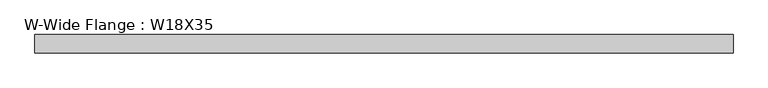
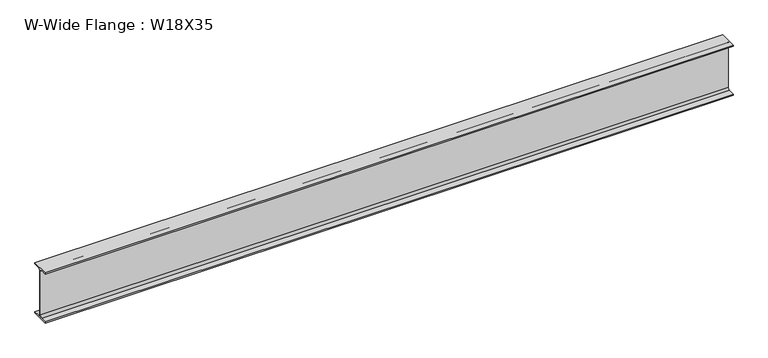
"""IFC4 building model written with IfcOpenShell, lengths in millimetres: beam geometry, W-Wide Flange : W18X35."""

from ifc_helpers import new_model, si_unit, point, frame, frame_2d, origin, place, context, project, spatial, polyline, circle_curve, trimmed, segment, composite_curve, outline, extrude, source, transform, mapped, element, save


def w_wide_flange_w18x35_b483a2b8(model_context):
    return source(origin(), model_context, "Body", "SweptSolid", [
        extrude(outline(composite_curve([segment(polyline([(76.2, -213.995), (76.2, -224.79), (-76.2, -224.79), (-76.2, -213.995), (-21.59, -213.995)]), True, "CONTINUOUS"), segment(trimmed(circle_curve(frame_2d((-21.59, -196.215)), 17.78), [point((-21.59, -213.995))], [point((-3.81, -196.215))], True, "CARTESIAN"), True, "CONTINUOUS"), segment(polyline([(-3.81, -196.215), (-3.81, 196.215)]), True, "CONTINUOUS"), segment(trimmed(circle_curve(frame_2d((-21.59, 196.215)), 17.78), [point((-3.81, 196.215))], [point((-21.59, 213.995))], True, "CARTESIAN"), True, "CONTINUOUS"), segment(polyline([(-21.59, 213.995), (-76.2, 213.995), (-76.2, 224.79), (76.2, 224.79), (76.2, 213.995), (21.59, 213.995)]), True, "CONTINUOUS"), segment(trimmed(circle_curve(frame_2d((21.59, 196.215)), 17.78), [point((21.59, 213.995))], [point((3.81, 196.215))], True, "CARTESIAN"), True, "CONTINUOUS"), segment(polyline([(3.81, 196.215), (3.81, -196.215)]), True, "CONTINUOUS"), segment(trimmed(circle_curve(frame_2d((21.59, -196.215)), 17.78), [point((3.81, -196.215))], [point((21.59, -213.995))], True, "CARTESIAN"), True, "CONTINUOUS"), segment(polyline([(21.59, -213.995), (76.2, -213.995)]), True, "CONTINUOUS")], self_intersect=False)), frame((-2921.0, 0.0, 0.0), z_axis=(1.0, 0.0, 0.0), x_axis=(0.0, 1.0, 0.0)), (0.0, 0.0, 1.0), 5842.0),
    ])


if __name__ == "__main__":
    model = new_model("IFC4")
    model_context = context("Model", 3, world=origin())
    ifc_project = project(units=[si_unit("LENGTHUNIT", "METRE", prefix="MILLI")], contexts=[model_context])
    site = spatial("IfcSite", under=ifc_project)
    building = spatial("IfcBuilding", under=site)
    placement = place(None, origin())
    w_wide_flange_w18x35_shape = w_wide_flange_w18x35_b483a2b8(model_context)
    element("IfcBeam", 1, ObjectType="W-Wide Flange : W18X35", at=placement, inside=building, context=model_context, shape_type="MappedRepresentation", body=[
        mapped(w_wide_flange_w18x35_shape, transform((0.0, 0.0, 0.0), x_axis=(1.0, 0.0, 0.0), y_axis=(0.0, 1.0, 0.0), z_axis=(0.0, 0.0, 1.0))),
    ])
    save(model, "model.ifc")

# Revit data of these elements
# Type "W-Wide Flange : W18X35"
#   Assembly Code = "B10"
#   W = 35
#   Length [instance default] = 5' - 0"
#   bf = 0' - 6"
#   d = 1' - 5.7"
#   k = 0' - 1 1/8"
#   k2 = 0' - 0.7"
#   tf = 0' - 0.425"
#   tw = 0' - 0.3"
#   A = 0.0715278 SF
#   Structural Material [instance default] = Steel ASTM A992
# Element 1 (IfcBeam, "W-Wide Flange : W18X35")
#   Structural Material = Steel ASTM A36
#   Materials on its faces: "Steel ASTM A36"
# Materials
#   "Steel ASTM A992": class "Metal", colour RGB 199 199 199, transparency 0, Description = "Structural steel 50ksi", Cost = 0
#   "Steel ASTM A36": class "Metal", colour RGB 199 199 199, transparency 0, Description = "Structural steel, ASTM A36 Grade B, mill finish", Cost = 0
